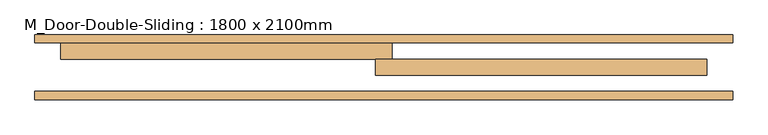
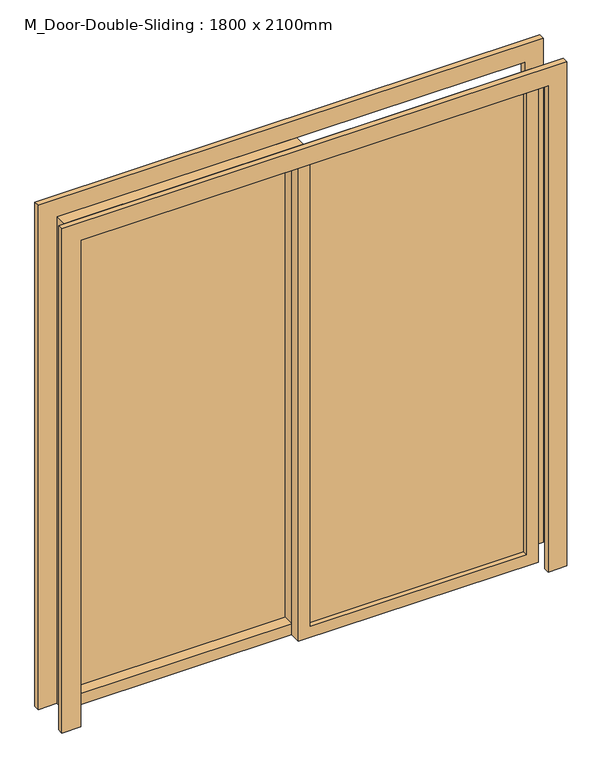
"""IFC4 building model written with IfcOpenShell, lengths in millimetres: door geometry, M_Door-Double-Sliding : 1800 x 2100mm."""

from ifc_helpers import new_model, si_unit, frame, origin, place, context, project, spatial, polyline, outline, extrude, source, transform, mapped, element, save


def m_door_double_sliding_1800_x_2100mm_1ba493e8(model_context):
    return source(origin(), model_context, "Body", "SweptSolid", [
        extrude(outline(polyline([(0.0, -1080.0), (0.0, -1000.0), (2200.0, -1000.0), (2200.0, 1000.0), (0.0, 1000.0), (0.0, 1080.0), (2280.0, 1080.0), (2280.0, -1080.0), (0.0, -1080.0)])), frame((0.0, 27.0, 0.0), z_axis=(0.0, 1.0, 0.0), x_axis=(0.0, 0.0, 1.0)), (0.0, 0.0, 1.0), 25.0),
        extrude(outline(polyline([(0.0, 1080.0), (2280.0, 1080.0), (2280.0, -1080.0), (0.0, -1080.0), (0.0, -1000.0), (2200.0, -1000.0), (2200.0, 1000.0), (0.0, 1000.0), (0.0, 1080.0)])), frame((0.0, 202.0, 0.0), z_axis=(0.0, 1.0, 0.0), x_axis=(0.0, 0.0, 1.0)), (0.0, 0.0, 1.0), 25.0),
        extrude(outline(polyline([(2200.0, -25.0), (0.0, -25.0), (0.0, 1000.0), (2200.0, 1000.0), (2200.0, -25.0)]), holes=[polyline([(2150.0, 25.0), (2150.0, 950.0), (50.0, 950.0), (50.0, 25.0), (2150.0, 25.0)])]), frame((0.0, 102.0, 0.0), z_axis=(0.0, 1.0, 0.0), x_axis=(0.0, 0.0, 1.0)), (0.0, 0.0, 1.0), 50.0),
        extrude(outline(polyline([(2200.0, 25.0), (2200.0, -1000.0), (0.0, -1000.0), (0.0, 25.0), (2200.0, 25.0)]), holes=[polyline([(2150.0, -25.0), (50.0, -25.0), (50.0, -950.0), (2150.0, -950.0), (2150.0, -25.0)])]), frame((0.0, 152.0, 0.0), z_axis=(0.0, 1.0, 0.0), x_axis=(0.0, 0.0, 1.0)), (0.0, 0.0, 1.0), 50.0),
        extrude(outline(polyline([(25.0, 130.175), (950.0, 130.175), (950.0, 123.825), (25.0, 123.825), (25.0, 130.175)])), frame((0.0, 0.0, 50.0), z_axis=(0.0, 0.0, 1.0), x_axis=(1.0, 0.0, 0.0)), (0.0, 0.0, 1.0), 2100.0),
        extrude(outline(polyline([(-25.0, 200.025), (-950.0, 200.025), (-950.0, 206.375), (-25.0, 206.375), (-25.0, 200.025)])), frame((0.0, 0.0, 50.0), z_axis=(0.0, 0.0, 1.0), x_axis=(1.0, 0.0, 0.0)), (0.0, 0.0, 1.0), 2100.0),
    ])


if __name__ == "__main__":
    model = new_model("IFC4")
    model_context = context("Model", 3, world=origin())
    ifc_project = project(units=[si_unit("LENGTHUNIT", "METRE", prefix="MILLI")], contexts=[model_context])
    site = spatial("IfcSite", under=ifc_project)
    building = spatial("IfcBuilding", under=site)
    placement = place(None, origin())
    m_door_double_sliding_1800_x_2100mm_shape = m_door_double_sliding_1800_x_2100mm_1ba493e8(model_context)
    element("IfcDoor", 1, ObjectType="M_Door-Double-Sliding : 1800 x 2100mm", at=placement, inside=building, context=model_context, shape_type="MappedRepresentation", body=[
        mapped(m_door_double_sliding_1800_x_2100mm_shape, transform((0.0, 0.0, 0.0), x_axis=(1.0, 0.0, 0.0), y_axis=(0.0, 1.0, 0.0), z_axis=(0.0, 0.0, 1.0))),
    ])
    save(model, "model.ifc")

# Revit data of these elements
# Type "M_Door-Double-Sliding : 1800 x 2100mm"
#   Type Mark = "23"
#   Construction Type Id = "opn-d45"
#   Assembly Code = "C1020"
#   Analytic Construction = "Wood frame, double glass door "
#   Thickness = 0.05 m
#   Thermal Resistance (R) = 0.31964 (m²·K)/W
#   Heat Transfer Coefficient (U) = 3.12872 W/(m²·K)
#   Height = 2.2 m
#   Rail Width = 0.05 m
#   Stiles = 0.05 m
#   Trim Projection Ext = 0.025 m
#   Trim Projection Int = 0.025 m
#   Trim Width = 0.08 m
#   Width = 2 m
#   Glazing = Glass
#   Panel Material = Wood - Birch - Solid Stained Light Low Gloss
#   Trim Material = Paint - Sienna
#   Visual Light Transmittance = 0
#   Solar Heat Gain Coefficient = 0
#   Function = (empty or 0)
#   Wall Closure = (empty or 0)
# Element 1 (IfcDoor, "M_Door-Double-Sliding : 1800 x 2100mm")
#   Materials on its faces: "Paint - Sienna", "Wood - Birch - Solid Stained Light Low Gloss", "Glass"
# Materials
#   "Glass": class "Glass", colour RGB 218 227 224, transparency 0.85, Description = "Soda Lime Glass", Cost = 0
#   "Wood - Birch - Solid Stained Light Low Gloss": class "Wood", colour RGB 227 170 128, transparency 0, Cost = 0
#   "Paint - Sienna": class "Miscellaneous", colour RGB 118 70 51, transparency 0, Cost = 0
